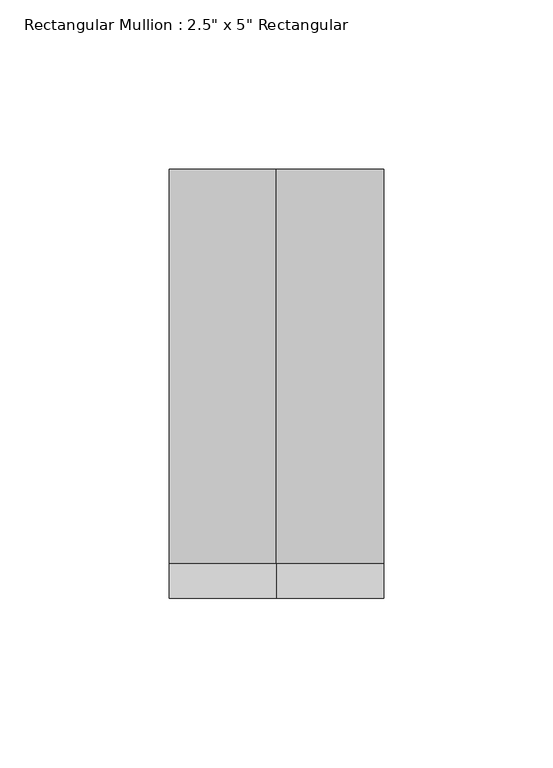
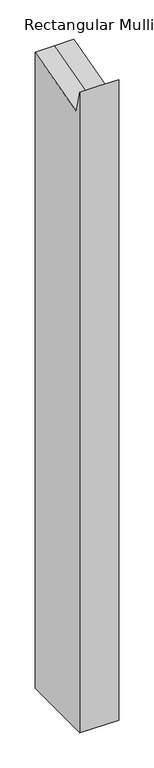
"""IFC4 building model written with IfcOpenShell, lengths in millimetres: member geometry."""

import ifcopenshell
import ifcopenshell.guid

model = None  # the IFC model being written
_history = None  # IfcOwnerHistory: only IFC2X3 demands one
_inside = {}  # id of a spatial element -> (the spatial element, [elements in it])
_under = {}  # id of a project, library or spatial element -> (it, [spatial elements below it])
_declared = {}  # id of a project -> (the project, [libraries it declares])
_typed = {}  # id of a type object -> (the type object, [elements of that type])
_made_of = {}  # id of a material, layer set ... -> (it, [elements and type objects made of it])


def new_model(schema):
    """Start an empty IFC model of exactly this schema.

    Asked for "IFC4X3", IfcOpenShell would pick the latest addendum, in which some entities
    have other attributes; the version numbers below select the first issue.
    IFC2X3 requires an IfcOwnerHistory on every rooted entity: one is made here for all.
    """
    global model, _history
    if schema == "IFC4X3":
        model = ifcopenshell.file(schema_version=(4, 3, 0, 0))
    else:
        model = ifcopenshell.file(schema=schema)
    _inside.clear()
    _under.clear()
    _declared.clear()
    _typed.clear()
    _made_of.clear()
    _history = None
    if model.schema == "IFC2X3":
        org = make("IfcOrganization", Name="unknown")
        user = make(
            "IfcPersonAndOrganization",
            ThePerson=make("IfcPerson", FamilyName="unknown"),
            TheOrganization=org,
        )
        app = make(
            "IfcApplication",
            ApplicationDeveloper=org,
            Version="unknown",
            ApplicationFullName="unknown",
            ApplicationIdentifier="unknown",
        )
        _history = make(
            "IfcOwnerHistory",
            OwningUser=user,
            OwningApplication=app,
            ChangeAction="ADDED",
            CreationDate=0,
        )
    return model


def make(cls, **values):
    """One entity of the class cls with the attributes given. An attribute that is None is left unset."""
    return model.create_entity(
        cls, **{name: value for name, value in values.items() if value is not None}
    )


def rooted(cls, **values):
    """An entity with a GlobalId (a new one), such as an element, a storey or a relation."""
    return make(cls, GlobalId=ifcopenshell.guid.new(), OwnerHistory=_history, **values)


def si_unit(unit_type, name, prefix=None):
    """IfcSIUnit, for example si_unit("LENGTHUNIT", "METRE", prefix="MILLI")."""
    return make("IfcSIUnit", UnitType=unit_type, Prefix=prefix, Name=name)


def assignment(units):
    """IfcUnitAssignment: the units of a project."""
    return None if units is None else make("IfcUnitAssignment", Units=units)


def point(xyz):
    """IfcCartesianPoint."""
    return None if xyz is None else make("IfcCartesianPoint", Coordinates=xyz)


def direction(xyz):
    """IfcDirection."""
    return None if xyz is None else make("IfcDirection", DirectionRatios=xyz)


def frame(location, z_axis=None, x_axis=None):
    """IfcAxis2Placement3D, a coordinate frame: its origin and axes. An axis left out is left unset."""
    return make(
        "IfcAxis2Placement3D",
        Location=point(location),
        Axis=direction(z_axis),
        RefDirection=direction(x_axis),
    )


def origin():
    """The frame at (0, 0, 0) with its axes left unset."""
    return frame((0.0, 0.0, 0.0))


def place(relative_to, where):
    """IfcLocalPlacement: puts the frame where relative to a parent placement (None: the world)."""
    return make(
        "IfcLocalPlacement", PlacementRelTo=relative_to, RelativePlacement=where
    )


def context(
    kind, dimensions, precision=None, world=None, true_north=None, identifier=None
):
    """IfcGeometricRepresentationContext, for example the 3D "Model" context."""
    return make(
        "IfcGeometricRepresentationContext",
        ContextIdentifier=identifier,
        ContextType=kind,
        CoordinateSpaceDimension=dimensions,
        Precision=precision,
        WorldCoordinateSystem=world,
        TrueNorth=true_north,
    )


def project(units=None, contexts=None):
    """IfcProject with its units and contexts."""
    return rooted(
        "IfcProject",
        Name="project",
        RepresentationContexts=contexts,
        UnitsInContext=assignment(units),
    )


def spatial(cls, under=None, at=None, **own):
    """A site, building, storey or space (cls), placed at a placement, below another one or the project."""
    s = rooted(cls, ObjectPlacement=at, **own)
    if under is not None:
        _under.setdefault(under.id(), (under, []))[1].append(s)
    return s


def faces_of(points, faces, orient=None, outer=None):
    """IfcFace entities. A face is a list of loops; a loop is a list of indices into points, from 0.

    orient and outer hold one flag for each loop. By default every Orientation is true, the
    first loop of a face is its IfcFaceOuterBound and the others are IfcFaceBound.
    """
    made = []
    for i, loops in enumerate(faces):
        bounds = []
        for j, loop in enumerate(loops):
            is_outer = j == 0 if outer is None else outer[i][j]
            bounds.append(
                make(
                    "IfcFaceOuterBound" if is_outer else "IfcFaceBound",
                    Bound=make("IfcPolyLoop", Polygon=[points[k] for k in loop]),
                    Orientation=True if orient is None else orient[i][j],
                )
            )
        made.append(make("IfcFace", Bounds=bounds))
    return made


def faceted_brep(points, faces, orient=None, outer=None, voids=None):
    """IfcFacetedBrep: a solid bounded by flat faces; with voids (closed shells), ...WithVoids."""
    shared = [point(p) for p in points]
    hull = make("IfcClosedShell", CfsFaces=faces_of(shared, faces, orient, outer))
    if voids is None:
        return make("IfcFacetedBrep", Outer=hull)
    return make(
        "IfcFacetedBrepWithVoids",
        Outer=hull,
        Voids=[
            make(cls, CfsFaces=faces_of(shared, fs, o, b)) for cls, fs, o, b in voids
        ],
    )


def shape(context_of_items, identifier, shape_type, items):
    """IfcShapeRepresentation: the items that make up one representation, for example the "Body"."""
    return make(
        "IfcShapeRepresentation",
        ContextOfItems=context_of_items,
        RepresentationIdentifier=identifier,
        RepresentationType=shape_type,
        Items=items,
    )


def source(mapping_origin, context_of_items, identifier, shape_type, items):
    """IfcRepresentationMap: a shape defined once, which mapped items show again and again."""
    return make(
        "IfcRepresentationMap",
        MappingOrigin=mapping_origin,
        MappedRepresentation=shape(context_of_items, identifier, shape_type, items),
    )


def transform(
    local_origin,
    x_axis=None,
    y_axis=None,
    z_axis=None,
    scale=None,
    scale2=None,
    scale3=None,
    uniform=True,
):
    """IfcCartesianTransformationOperator3D, or its non-uniform kind. x_axis, y_axis, z_axis: its Axis1, 2, 3."""
    if uniform:
        return make(
            "IfcCartesianTransformationOperator3D",
            Axis1=direction(x_axis),
            Axis2=direction(y_axis),
            LocalOrigin=point(local_origin),
            Scale=scale,
            Axis3=direction(z_axis),
        )
    return make(
        "IfcCartesianTransformationOperator3DnonUniform",
        Axis1=direction(x_axis),
        Axis2=direction(y_axis),
        LocalOrigin=point(local_origin),
        Scale=scale,
        Axis3=direction(z_axis),
        Scale2=scale2,
        Scale3=scale3,
    )


def mapped(mapping_source, mapping_target):
    """IfcMappedItem: shows the shape of a source again, moved by a transform."""
    return make(
        "IfcMappedItem", MappingSource=mapping_source, MappingTarget=mapping_target
    )


def made_of(thing, what):
    """Note that an element or type object is made of a material, layer set ...; save() writes the relation."""
    if what is not None:
        _made_of.setdefault(what.id(), (what, []))[1].append(thing)
    return thing


def element(
    cls,
    number,
    at=None,
    inside=None,
    cuts=None,
    type_object=None,
    material=None,
    context=None,
    identifier="Body",
    shape_type=None,
    held_by="IfcProductDefinitionShape",
    body=None,
    shapes=None,
    **own,
):
    """One element of the class cls, such as IfcWall. Its Tag is "e" and its number.

    at: its placement. inside: the storey or other place that contains it. cuts: it is an
    opening in that element (IfcRelVoidsElement). A single representation is given by context,
    identifier, shape_type and body (its items); several are given by shapes. held_by: the class
    of the entity that holds the representations. save() writes the other relations.
    """
    e = rooted(cls, Tag="e%d" % number, ObjectPlacement=at, **own)
    if body is not None:
        shapes = [shape(context, identifier, shape_type, body)]
    if shapes is not None:
        e.Representation = make(held_by, Representations=shapes)
    if inside is not None:
        _inside.setdefault(inside.id(), (inside, []))[1].append(e)
    if cuts is not None:
        rooted(
            "IfcRelVoidsElement", RelatingBuildingElement=cuts, RelatedOpeningElement=e
        )
    if type_object is not None:
        _typed.setdefault(type_object.id(), (type_object, []))[1].append(e)
    return made_of(e, material)


def aggregate(whole, parts):
    """IfcRelAggregates: a whole, such as a stair, and the parts it consists of."""
    return rooted("IfcRelAggregates", RelatingObject=whole, RelatedObjects=parts)


def save(model, path):
    """Write the relations noted so far, then the file.

    IfcRelAggregates (storeys below a building ...), IfcRelContainedInSpatialStructure (elements
    in a storey), IfcRelDefinesByType, IfcRelAssociatesMaterial and IfcRelDeclares: one each for
    every whole, place, type object, material and project.
    """
    for whole, parts in _under.values():
        aggregate(whole, parts)
    for where, things in _inside.values():
        rooted(
            "IfcRelContainedInSpatialStructure",
            RelatedElements=things,
            RelatingStructure=where,
        )
    for kind, things in _typed.values():
        rooted("IfcRelDefinesByType", RelatedObjects=things, RelatingType=kind)
    for what, things in _made_of.values():
        rooted("IfcRelAssociatesMaterial", RelatedObjects=things, RelatingMaterial=what)
    for by, libraries in _declared.values():
        rooted("IfcRelDeclares", RelatingContext=by, RelatedDefinitions=libraries)
    model.write(path)


def member_64534d09(model_context):
    return source(origin(), model_context, "Body", "Brep", [
        faceted_brep([(31.75, 63.5, -1088.0706742), (31.75, -63.5, -1088.0706742), (-31.75, -63.5, -1088.0706742), (-31.75, 63.5, -1088.0706742), (-31.75, 63.5, 15.894755), (0.0, 63.5, 15.894755), (31.75, 63.5, 15.894755), (-31.75, -63.5, 23.3900664), (-31.75, -53.1187853, -15.3531543), (31.75, -63.5, 23.3900664), (0.0, -63.5, 23.3900664), (31.75, -53.1187853, -15.3531543), (0.0, -53.1187853, -15.3531543)], [[[0, 1, 2, 3]], [[4, 5, 6, 0, 3]], [[7, 8, 4, 3, 2]], [[9, 10, 7, 2, 1]], [[6, 11, 9, 1, 0]], [[6, 5, 12, 11]], [[5, 4, 8, 12]], [[8, 7, 10, 12]], [[10, 9, 11, 12]]]),
    ])


if __name__ == "__main__":
    model = new_model("IFC4")
    model_context = context("Model", 3, world=origin())
    ifc_project = project(units=[si_unit("LENGTHUNIT", "METRE", prefix="MILLI")], contexts=[model_context])
    site = spatial("IfcSite", under=ifc_project)
    building = spatial("IfcBuilding", under=site)
    placement = place(None, origin())
    member_shape = member_64534d09(model_context)
    element("IfcMember", 1, ObjectType="Rectangular Mullion : 2.5\" x 5\" Rectangular", at=placement, inside=building, context=model_context, shape_type="MappedRepresentation", body=[
        mapped(member_shape, transform((0.0, 0.0, 0.0), x_axis=(1.0, 0.0, 0.0), y_axis=(0.0, 1.0, 0.0), z_axis=(0.0, 0.0, 1.0))),
    ])
    save(model, "model.ifc")

# Revit data of these elements
# Project information
#   Project Issue Date = "Issue Date"
#   Project Status = "Project Status"
#   Client Name = "Owner"
#   Project Address = "Enter address here"
#   Project Name = "Project Name"
#   Project Number = "Project Number"
# Type "Rectangular Mullion : 2.5\" x 5\" Rectangular"
#   built-in parameter 1007304 = 0.416667 (stored number, unit not read)
#   built-in parameter 1007301 = 0.104167 (stored number, unit not read)
#   built-in parameter 1007300 = 0.104167 (stored number, unit not read)
# Element 1 (IfcMember, "Rectangular Mullion : 2.5\" x 5\" Rectangular")
#   Materials on its faces: "Aluminum"
# Materials
#   "Aluminum": class "Metal", colour RGB 247 247 247, transparency 0, Description = "Aluminum 6061", Cost = 0
